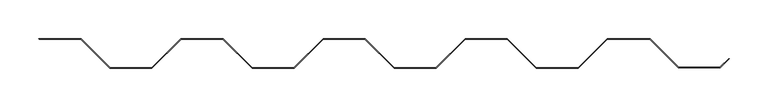
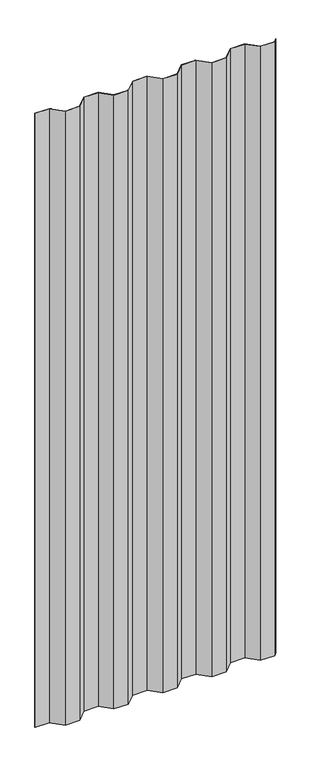
"""IFC4 building model written with IfcOpenShell, lengths in millimetres: proxy geometry, MBCI 7.2-V Panel3 : MBCI 7.2-V Panel-1."""

from ifc_helpers import new_model, si_unit, frame, origin, place, context, project, spatial, polyline, outline, extrude, source, transform, mapped, element, save


def generic_models_0e9549c0(model_context):
    return source(origin(), model_context, "Body", "SweptSolid", [
        extrude(outline(polyline([(587418.0082638, -531601.7259841), (587364.5694989, -531601.7259841), (587363.9741864, -531601.1306716), (587418.2548503, -531601.1306716), (587455.7452503, -531638.6210716), (587509.3637864, -531638.6210716), (587546.8541864, -531601.1306716), (587601.1348503, -531601.1306716), (587638.6252503, -531638.6210716), (587692.2437864, -531638.6210716), (587729.7341864, -531601.1306716), (587784.0148503, -531601.1306716), (587821.5052503, -531638.6210716), (587875.1237864, -531638.6210716), (587912.6141864, -531601.1306716), (587966.8948503, -531601.1306716), (588004.3852503, -531638.6210716), (588058.0037864, -531638.6210716), (588095.4941864, -531601.1306716), (588150.6384503, -531601.1306716), (588187.5192503, -531638.0114716), (588240.6073773, -531638.0114716), (588251.7378112, -531626.8810377), (588252.5246865, -531626.9360614), (588240.8539638, -531638.6067841), (588187.2726638, -531638.6067841), (588150.3918638, -531601.7259841), (588095.7407729, -531601.7259841), (588058.2503729, -531639.2163841), (588004.1386638, -531639.2163841), (587966.6482638, -531601.7259841), (587912.8607729, -531601.7259841), (587875.3703729, -531639.2163841), (587821.2586638, -531639.2163841), (587783.7682638, -531601.7259841), (587729.9807729, -531601.7259841), (587692.4903729, -531639.2163841), (587638.3786638, -531639.2163841), (587600.8882638, -531601.7259841), (587547.1007729, -531601.7259841), (587509.6103729, -531639.2163841), (587455.4986638, -531639.2163841), (587418.0082638, -531601.7259841)])), frame((0.0, 0.0, 6.35), z_axis=(0.0, 0.0, 1.0), x_axis=(1.0, 0.0, 0.0)), (0.0, 0.0, 1.0), 2432.05),
    ])


if __name__ == "__main__":
    model = new_model("IFC4")
    model_context = context("Model", 3, world=origin())
    ifc_project = project(units=[si_unit("LENGTHUNIT", "METRE", prefix="MILLI")], contexts=[model_context])
    site = spatial("IfcSite", under=ifc_project)
    building = spatial("IfcBuilding", under=site)
    placement = place(None, origin())
    generic_models_shape = generic_models_0e9549c0(model_context)
    element("IfcBuildingElementProxy", 1, Name="MBCI 7.2-V Panel3 : MBCI 7.2-V Panel-1", ObjectType="MBCI 7.2-V Panel3 : MBCI 7.2-V Panel-1", at=placement, inside=building, context=model_context, shape_type="MappedRepresentation", body=[
        mapped(generic_models_shape, transform((0.0, 0.0, 0.0), x_axis=(1.0, 0.0, 0.0), y_axis=(0.0, 1.0, 0.0), z_axis=(0.0, 0.0, 1.0))),
    ])
    save(model, "model.ifc")

# Revit data of these elements
# Element 1 (IfcBuildingElementProxy, "MBCI 7.2-V Panel3 : MBCI 7.2-V Panel-1")
#   Materials on its faces: "MTL PANEL"
# Materials
#   "MTL PANEL": class "Generic", colour RGB 239 242 240, transparency 0, Cost = 0
